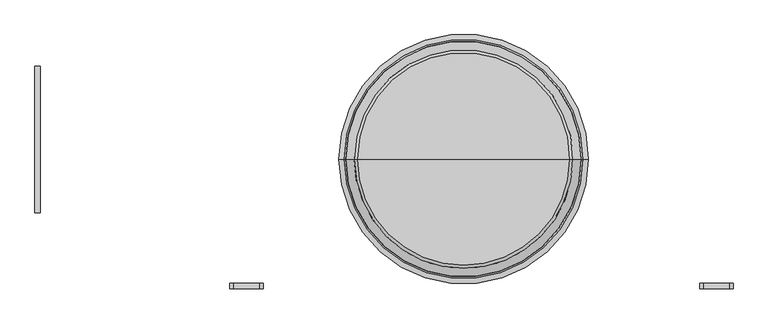
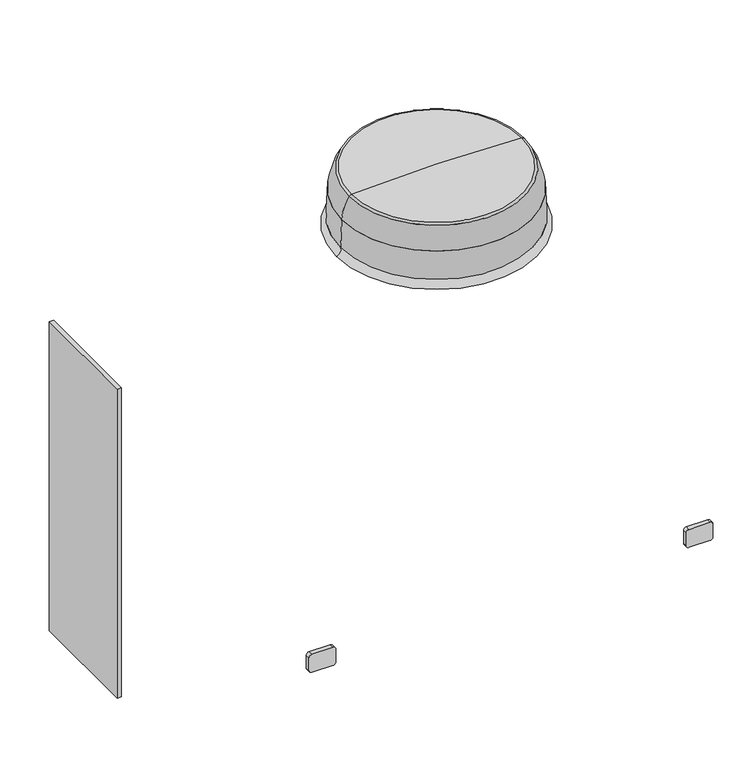
"""IFC4 building model written with IfcOpenShell, lengths in millimetres: proxy geometry, PURY-P168-288_YSJMU_Heat_Recovery_460V : PURY-P192YSJMU-A(-BS)_460V."""

from ifc_helpers import new_model, si_unit, point, frame, frame_2d, origin, place, context, project, spatial, polyline, circle_curve, ellipse_curve, trimmed, segment, composite_curve, outline, extrude, source, transform, mapped, element, save
from ifc_brep_helpers import plane_surface, revolved_surface, advanced_brep


def mechanical_equipment_79fc2163(model_context):
    return source(origin(), model_context, "Body", "SolidModel", [
        extrude(outline(polyline([(-748.962, -164.0), (-748.962, 284.0), (-732.962, 284.0), (-732.962, -164.0), (-748.962, -164.0)])), frame((0.0, 0.0, 54.0), z_axis=(0.0, 0.0, 1.0), x_axis=(1.0, 0.0, 0.0)), (0.0, 0.0, 1.0), 1245.8),
        advanced_brep(
        [(202.9156536, 0.0, 1550.0000157), (924.1603464, 0.0, 1550.0000157), (563.538, 0.0, 1550.0000157), (228.7569245, 0.0, 1635.7196156), (898.3190755, 0.0, 1635.7196156), (237.9260831, 0.0, 1640.2981249), (889.1499169, 0.0, 1640.2981249), (563.538, 0.0, 1649.7941679)],
        [
            (0, 1, circle_curve(frame((563.538, 0.0, 1550.0000157), z_axis=(0.0, 0.0, -1.0), x_axis=(1.0, 0.0, 0.0)), 360.6223464)),
            (1, 2),
            (2, 0),
            (1, 0, circle_curve(frame((563.538, 0.0, 1550.0000157), z_axis=(0.0, 0.0, -1.0), x_axis=(1.0, 0.0, 0.0)), 360.6223464)),
            (3, 4, circle_curve(frame((563.538, 0.0, 1635.7196156), z_axis=(0.0, 0.0, -1.0), x_axis=(1.0, 0.0, 0.0)), 334.7810755)),
            (4, 1, circle_curve(frame((740.2568175, 0.0, 1541.3148332), z_axis=(0.0, 1.0, 0.0), x_axis=(1.0, 0.0, 0.0)), 184.1085015)),
            (0, 3, circle_curve(frame((386.8191825, 0.0, 1541.3148332), z_axis=(0.0, 1.0, 0.0), x_axis=(-1.0, 0.0, 0.0)), 184.1085015)),
            (4, 3, circle_curve(frame((563.538, 0.0, 1635.7196156), z_axis=(0.0, 0.0, -1.0), x_axis=(1.0, 0.0, 0.0)), 334.7810755)),
            (5, 6, circle_curve(frame((563.538, 0.0, 1640.2981249), z_axis=(0.0, 0.0, -1.0), x_axis=(1.0, 0.0, 0.0)), 325.6119169)),
            (6, 4, circle_curve(frame((889.1499169, 0.0, 1628.8275558), z_axis=(0.0, 1.0, 0.0), x_axis=(1.0, 0.0, 0.0)), 11.4705691)),
            (3, 5, circle_curve(frame((237.9260831, 0.0, 1628.8275558), z_axis=(0.0, 1.0, 0.0), x_axis=(-1.0, 0.0, 0.0)), 11.4705691)),
            (6, 5, circle_curve(frame((563.538, 0.0, 1640.2981249), z_axis=(0.0, 0.0, -1.0), x_axis=(1.0, 0.0, 0.0)), 325.6119169)),
            (7, 6, circle_curve(frame((563.538, 0.0, -3937.4433334), z_axis=(0.0, 1.0, 0.0), x_axis=(1.0, 0.0, 0.0)), 5587.2375013)),
            (5, 7, circle_curve(frame((563.538, 0.0, -3937.4433334), z_axis=(0.0, 1.0, 0.0), x_axis=(-1.0, 0.0, 0.0)), 5587.2375013)),
        ],
        [
            plane_surface(frame((563.538, 0.0, 1550.0000157), z_axis=(0.0, 0.0, -1.0), x_axis=(1.0, 0.0, 0.0))),
            revolved_surface(trimmed(ellipse_curve(frame((740.2568175, 0.0, 1541.3148332), z_axis=(0.0, -1.0, 0.0), x_axis=(1.0, 0.0, 0.0)), 184.1085015, 184.1085015), [point((924.1603464, 0.0, 1550.0000157))], [point((898.3190755, 0.0, 1635.7196156))], True, "CARTESIAN"), (563.538, 0.0, 1605.0), (0.0, 0.0, 1.0)),
            revolved_surface(trimmed(ellipse_curve(frame((889.1499169, 0.0, 1628.8275558), z_axis=(0.0, -1.0, 0.0), x_axis=(1.0, 0.0, 0.0)), 11.4705691, 11.4705691), [point((898.3190755, 0.0, 1635.7196156))], [point((889.1499169, 0.0, 1640.2981249))], True, "CARTESIAN"), (563.538, 0.0, 1605.0), (0.0, 0.0, 1.0)),
            revolved_surface(trimmed(ellipse_curve(frame((563.538, 0.0, -3937.4433334), z_axis=(0.0, -1.0, 0.0), x_axis=(1.0, 0.0, 0.0)), 5587.2375013, 5587.2375013), [point((889.1499169, 0.0, 1640.2981249))], [point((563.538, 0.0, 1649.7941679))], True, "CARTESIAN"), (563.538, 0.0, 1605.0), (0.0, 0.0, 1.0)),
        ],
        [
            (0, [[1, 2, 3]]),
            (0, [[4, -3, -2]]),
            (1, [[5, 6, -1, 7]]),
            (1, [[8, -7, -4, -6]]),
            (2, [[9, 10, -5, 11]]),
            (2, [[12, -11, -8, -10]]),
            (3, [[13, -9, 14]]),
            (3, [[-14, -12, -13]]),
        ],
    ),
        advanced_brep(
        [(181.4881528, 0.0, 1410.0), (945.5878472, 0.0, 1410.0), (563.538, 0.0, 1410.0), (198.0531583, 0.0, 1438.6914312), (929.0228417, 0.0, 1438.6914312), (202.9129453, 0.0, 1550.0000157), (924.1630547, 0.0, 1550.0000157), (563.538, 0.0, 1550.0000157)],
        [
            (0, 1, circle_curve(frame((563.538, 0.0, 1410.0), z_axis=(0.0, 0.0, -1.0), x_axis=(1.0, 0.0, 0.0)), 382.0498472)),
            (1, 2),
            (2, 0),
            (1, 0, circle_curve(frame((563.538, 0.0, 1410.0), z_axis=(0.0, 0.0, -1.0), x_axis=(1.0, 0.0, 0.0)), 382.0498472)),
            (3, 4, circle_curve(frame((563.538, 0.0, 1438.6914312), z_axis=(0.0, 0.0, -1.0), x_axis=(1.0, 0.0, 0.0)), 365.4848417)),
            (4, 1, circle_curve(frame((949.7748091, 0.0, 1431.5449644), z_axis=(0.0, -1.0, 0.0), x_axis=(1.0, 0.0, 0.0)), 21.9480327)),
            (0, 3, circle_curve(frame((177.3011909, 0.0, 1431.5449644), z_axis=(0.0, -1.0, 0.0), x_axis=(-1.0, 0.0, 0.0)), 21.9480327)),
            (4, 3, circle_curve(frame((563.538, 0.0, 1438.6914312), z_axis=(0.0, 0.0, -1.0), x_axis=(1.0, 0.0, 0.0)), 365.4848417)),
            (5, 6, circle_curve(frame((563.538, 0.0, 1550.0000157), z_axis=(0.0, 0.0, -1.0), x_axis=(1.0, 0.0, 0.0)), 360.6250547)),
            (6, 4),
            (3, 5),
            (6, 5, circle_curve(frame((563.538, 0.0, 1550.0000157), z_axis=(0.0, 0.0, -1.0), x_axis=(1.0, 0.0, 0.0)), 360.6250547)),
            (7, 6),
            (5, 7),
        ],
        [
            plane_surface(frame((563.538, 0.0, 1410.0), z_axis=(0.0, 0.0, -1.0), x_axis=(1.0, 0.0, 0.0))),
            revolved_surface(trimmed(ellipse_curve(frame((949.7748091, 0.0, 1431.5449644), z_axis=(0.0, 1.0, 0.0), x_axis=(1.0, 0.0, 0.0)), 21.9480327, 21.9480327), [point((945.5878472, 0.0, 1410.0))], [point((929.0228417, 0.0, 1438.6914312))], True, "CARTESIAN"), (563.538, 0.0, 1470.0), (0.0, 0.0, 1.0)),
            revolved_surface(polyline([(929.0228417, 0.0, 1438.6914312), (924.1630547, 0.0, 1550.0000157)]), (563.538, 0.0, 1470.0), (0.0, 0.0, 1.0)),
            plane_surface(frame((563.538, 0.0, 1550.0000157), z_axis=(0.0, 0.0, 1.0), x_axis=(1.0, 0.0, 0.0))),
        ],
        [
            (0, [[1, 2, 3]]),
            (0, [[4, -3, -2]]),
            (1, [[5, 6, -1, 7]]),
            (1, [[8, -7, -4, -6]]),
            (2, [[9, 10, -5, 11]]),
            (2, [[12, -11, -8, -10]]),
            (3, [[13, -9, 14]]),
            (3, [[-14, -12, -13]]),
        ],
    ),
        extrude(outline(composite_curve([segment(trimmed(circle_curve(frame_2d((148.5853631, 1296.6117511)), 9.9920268), [point((158.5773899, 1296.6117511))], [point((148.5853631, 1286.6197243))], False, "CARTESIAN"), True, "CONTINUOUS"), segment(polyline([(148.5853631, 1286.6197243), (96.5694168, 1286.6197243)]), True, "CONTINUOUS"), segment(trimmed(circle_curve(frame_2d((96.5694168, 1296.6117511)), 9.9920268), [point((96.5694168, 1286.6197243))], [point((86.5773899, 1296.6117511))], False, "CARTESIAN"), True, "CONTINUOUS"), segment(polyline([(86.5773899, 1296.6117511), (86.5773899, 1378.6276974)]), True, "CONTINUOUS"), segment(trimmed(circle_curve(frame_2d((96.5694168, 1378.6276974)), 9.9920268), [point((86.5773899, 1378.6276974))], [point((96.5694168, 1388.6197243))], False, "CARTESIAN"), True, "CONTINUOUS"), segment(polyline([(96.5694168, 1388.6197243), (148.5853631, 1388.6197243)]), True, "CONTINUOUS"), segment(trimmed(circle_curve(frame_2d((148.5853631, 1378.6276974)), 9.9920268), [point((148.5853631, 1388.6197243))], [point((158.5773899, 1378.6276974))], False, "CARTESIAN"), True, "CONTINUOUS"), segment(polyline([(158.5773899, 1378.6276974), (158.5773899, 1296.6117511)]), True, "CONTINUOUS")], self_intersect=False)), frame((0.0, -397.2710787, 0.0), z_axis=(0.0, 1.0, 0.0), x_axis=(0.0, 0.0, 1.0)), (0.0, 0.0, 1.0), 17.2710787),
        extrude(outline(composite_curve([segment(trimmed(circle_curve(frame_2d((148.5853631, -142.3882489)), 9.9920268), [point((158.5773899, -142.3882489))], [point((148.5853631, -152.3802757))], False, "CARTESIAN"), True, "CONTINUOUS"), segment(polyline([(148.5853631, -152.3802757), (96.5694168, -152.3802757)]), True, "CONTINUOUS"), segment(trimmed(circle_curve(frame_2d((96.5694168, -142.3882489)), 9.9920268), [point((96.5694168, -152.3802757))], [point((86.5773899, -142.3882489))], False, "CARTESIAN"), True, "CONTINUOUS"), segment(polyline([(86.5773899, -142.3882489), (86.5773899, -60.3723026)]), True, "CONTINUOUS"), segment(trimmed(circle_curve(frame_2d((96.5694168, -60.3723026)), 9.9920268), [point((86.5773899, -60.3723026))], [point((96.5694168, -50.3802757))], False, "CARTESIAN"), True, "CONTINUOUS"), segment(polyline([(96.5694168, -50.3802757), (148.5853631, -50.3802757)]), True, "CONTINUOUS"), segment(trimmed(circle_curve(frame_2d((148.5853631, -60.3723026)), 9.9920268), [point((148.5853631, -50.3802757))], [point((158.5773899, -60.3723026))], False, "CARTESIAN"), True, "CONTINUOUS"), segment(polyline([(158.5773899, -60.3723026), (158.5773899, -142.3882489)]), True, "CONTINUOUS")], self_intersect=False)), frame((0.0, -397.2710787, 0.0), z_axis=(0.0, 1.0, 0.0), x_axis=(0.0, 0.0, 1.0)), (0.0, 0.0, 1.0), 17.2710787),
    ])


if __name__ == "__main__":
    model = new_model("IFC4")
    model_context = context("Model", 3, world=origin())
    ifc_project = project(units=[si_unit("LENGTHUNIT", "METRE", prefix="MILLI")], contexts=[model_context])
    site = spatial("IfcSite", under=ifc_project)
    building = spatial("IfcBuilding", under=site)
    placement = place(None, origin())
    mechanical_equipment_shape = mechanical_equipment_79fc2163(model_context)
    element("IfcBuildingElementProxy", 1, Name="PURY-P168-288_YSJMU_Heat_Recovery_460V : PURY-P192YSJMU-A(-BS)_460V", ObjectType="PURY-P168-288_YSJMU_Heat_Recovery_460V : PURY-P192YSJMU-A(-BS)_460V", at=placement, inside=building, context=model_context, shape_type="MappedRepresentation", body=[
        mapped(mechanical_equipment_shape, transform((0.0, 0.0, 0.0), x_axis=(1.0, 0.0, 0.0), y_axis=(0.0, 1.0, 0.0), z_axis=(0.0, 0.0, 1.0))),
    ])
    save(model, "model.ifc")

# Revit data of these elements
# Type "PURY-P168-288_YSJMU_Heat_Recovery_460V : PURY-P192YSJMU-A(-BS)_460V"
#   Unit Weight (LBS) = "618 x 2"
#   Technical and Installation = "http://www.mrslim.com/customerCare/resources.asp"
#   Specification URL = "http://www.mrslim.com/customerCare/resources.asp"
#   Sound Pressure Levels (dB(A)) = "61"
#   SmartBIM Object Created By = "Reed Construction Data"
#   Refrigerant Type = "R410A"
#   Refrigerant Charge = ""
#   Recommended Breaker Size = "25 A x 1 + 15 A x 1"
#   Protection Devices Inverter = "Overheat / Overcurrent Protection"
#   Protection Devices High Pressure = "601 psi / 4.15 MPa"
#   Protection Devices Fan = "Overheat Protection / Thermal Switch"
#   Protection Devices Compressor = "Overheat Protection / Thermal Switch"
#   Product URL = "http://www.mrslim.com/customerCare/resources.asp"
#   Power Source = "208 / 230V, 3-phase, 60Hz"
#   Power Input Heating = "16.07 kW"
#   Power Input Cooling = "17.84 kW"
#   URL = "http://www.mehvac.com"
#   OmniClass Code = "22-23 81 26"
#   MOCP = "30 A x 1 + 15 A x 1"
#   MCA = "23 A x 1 + 13 A x 1"
#   Lubricant = "MEL32"
#   Installation URL = "http://www.mrslim.com/customerCare/resources.asp"
#   Heating Outdoor = "-4° ~ +60°F (-20° ~ +16°C) WB"
#   Heating Indoor = "59° ~ 81°F (15° ~ 27°C) DB"
#   Heating Capacity(BTU) = "215,000"
#   Fan Type x Quantity = "Propeller Fan x 3"
#   Fan Motor Output = "0.92 kW x 3"
#   Fan Air Flow Rate = "10,600 CFM x 1 / 6,180 CFM x 1"
#   Model = "PURY-P192YSJMU-A(-BS)_460V"
#   Manufacturer = "Mitsubishi Electric"
#   Current Heating = "28.2 A"
#   Current Cooling = "25.5 A"
#   Cooling Outdoor = "23° ~ 115°F (-5° ~ +46°C) DB"
#   Cooling Indoor = "59° ~ 75°F (15° ~ +24°C) WB"
#   Cooling Capacity (BTU) = "192,000"
#   Compressor Type x Quantity = "Inverter-driven Scroll Hermetic x 1 for Each Module"
#   Compressor Operating Range = "8% to 100%"
#   Case Heater = "0.045 kW"
#   Assembly Code = "D3090100"
#   95 CSI = "15740"
#   04 CSI = "23 81 26"
#   Voltage = 208 V
#   SmartBIM Object Version = 3
#   Refrigerant Pipe diameter (low pressure) = 28.575 mm
#   Refrigerant Pipe diameter (high pressure) = 22.225 mm
#   Phase = 3
#   Outdoor Unit2-Width = 920 mm
#   Outdoor Unit1-Width = 1750 mm
#   Offset = 30 mm
#   Hertz = 60
#   Height = 1650 mm
#   Depth = 760 mm
#   Apparent Load = 0 VA
#   Number of Poles = 2
#   Load Classification = Other
#   External Material = Pre-coated Galvanized-steel Sheets
#   External Finish = Pre-coated Galvanized-steel Sheets
#   Air Outlet Unit Material = Metal Grille
#   Air Inlet Unit Material = Grille
#   Type Comments = ""
#   Description = (empty or 0)
#   Default Elevation = 0
# Element 1 (IfcBuildingElementProxy, "PURY-P168-288_YSJMU_Heat_Recovery_460V : PURY-P192YSJMU-A(-BS)_460V")
#   Materials on its faces: "Pre-coated Galvanized-steel Sheets", "Grille", "Metal Grille"
# Materials
#   "Pre-coated Galvanized-steel Sheets": class "Metal", colour RGB 189 187 185, transparency 0
#   "Metal Grille": class "Metal", colour RGB 10 10 10, transparency 0
#   "Grille": class "Miscellaneous", colour RGB 0 0 0, transparency 0
